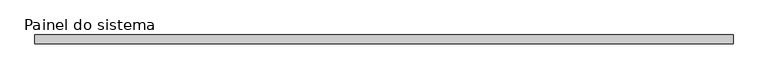
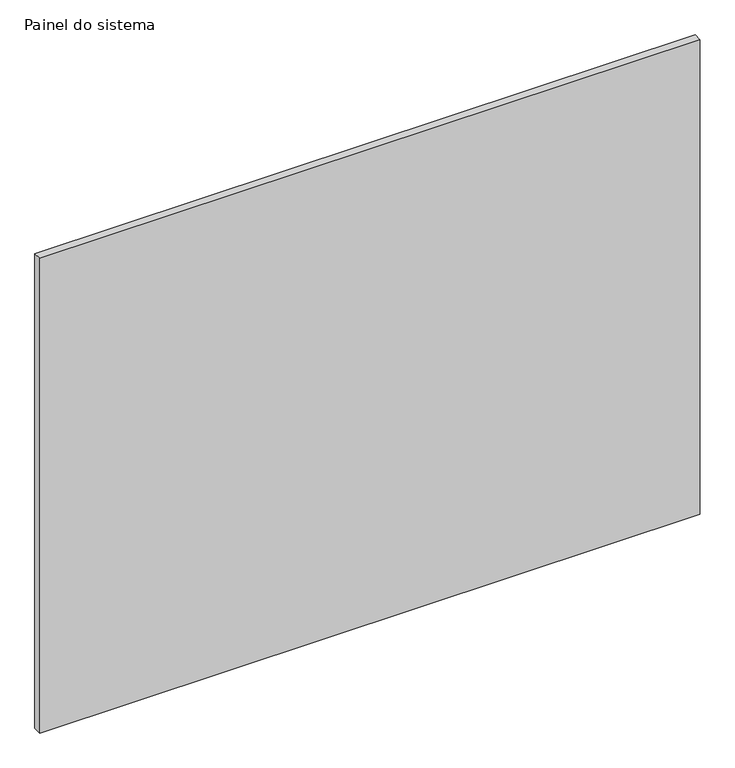
"""IFC4 building model written with IfcOpenShell, lengths in millimetres: plate geometry, Painel do sistema : Envidraçado."""

from ifc_helpers import new_model, si_unit, origin, origin_with_axes, place, context, project, spatial, polyline, outline, extrude, source, transform, mapped, element, save


def painel_do_sistema_fd15dc3a(model_context):
    return source(origin(), model_context, "Body", "SweptSolid", [
        extrude(outline(polyline([(987.5, 24.5), (-987.5, 24.5), (-987.5, 49.5), (987.5, 49.5), (987.5, 24.5)])), origin_with_axes(), (0.0, 0.0, 1.0), 1500.0),
    ])


if __name__ == "__main__":
    model = new_model("IFC4")
    model_context = context("Model", 3, world=origin())
    ifc_project = project(units=[si_unit("LENGTHUNIT", "METRE", prefix="MILLI")], contexts=[model_context])
    site = spatial("IfcSite", under=ifc_project)
    building = spatial("IfcBuilding", under=site)
    placement = place(None, origin())
    painel_do_sistema_shape = painel_do_sistema_fd15dc3a(model_context)
    element("IfcPlate", 1, ObjectType="Painel do sistema : Envidraçado", at=placement, inside=building, context=model_context, shape_type="MappedRepresentation", body=[
        mapped(painel_do_sistema_shape, transform((0.0, 0.0, 0.0), x_axis=(1.0, 0.0, 0.0), y_axis=(0.0, 1.0, 0.0), z_axis=(0.0, 0.0, 1.0))),
    ])
    save(model, "model.ifc")

# Revit data of these elements
# Type "Painel do sistema : Envidraçado"
#   Construction Type Id = "GSP4R"
#   Analytic Construction = "Vidraça única Pilkington 1/8 pol"
#   Visual Light Transmittance = 0.9
#   Solar Heat Gain Coefficient = 0.86
#   Heat Transfer Coefficient (U) = 6.7069 W/(m²·K)
# Element 1 (IfcPlate, "Painel do sistema : Envidraçado")
#   Materials on its faces: "Vidro"
# Materials
#   "Vidro": class "Vidro", colour RGB 0 128 192, transparency 0.9, Description = "Vidro de sílica", Cost = 0
